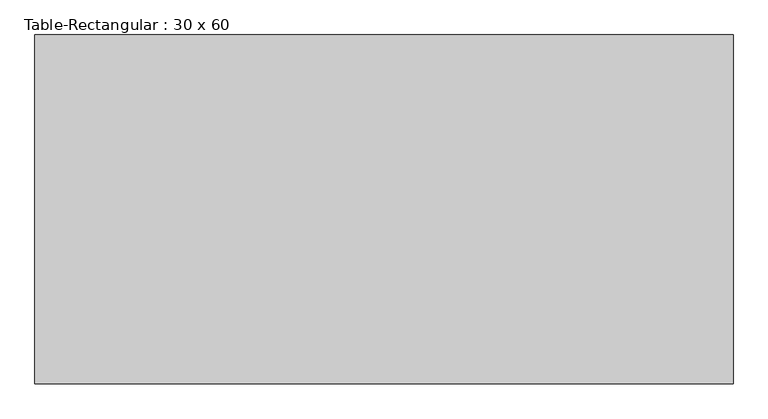
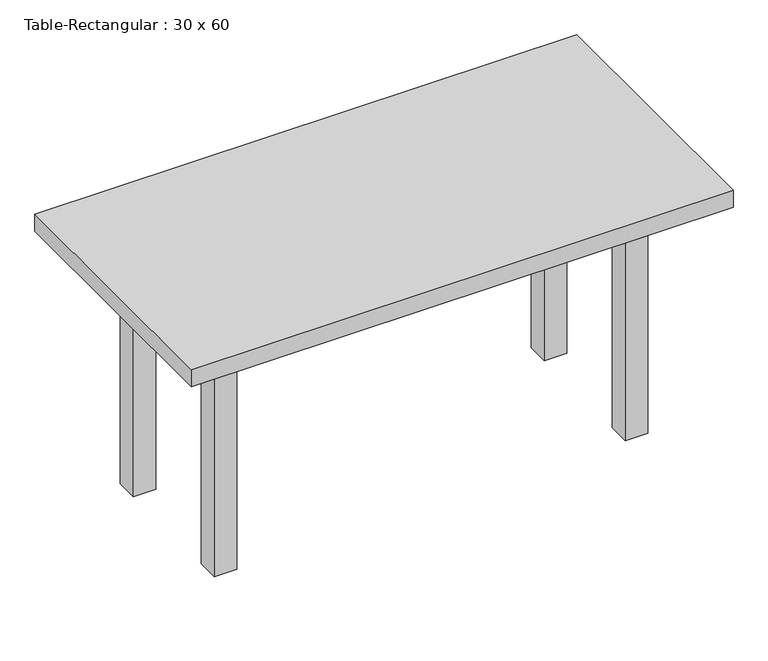
"""IFC4 building model written with IfcOpenShell, lengths in millimetres: furniture geometry, Table-Rectangular : 30 x 60."""

from ifc_helpers import new_model, si_unit, frame, origin, origin_with_axes, place, context, project, spatial, polyline, outline, extrude, source, transform, mapped, element, save


def table_rectangular_30_x_60_d900495b(model_context):
    return source(origin(), model_context, "Body", "SweptSolid", [
        extrude(outline(polyline([(546.1, 190.5), (546.1, 165.1), (-546.1, 165.1), (-546.1, 190.5), (546.1, 190.5)])), frame((0.0, 0.0, 609.6), z_axis=(0.0, 0.0, 1.0), x_axis=(1.0, 0.0, 0.0)), (0.0, 0.0, 1.0), 101.6),
        extrude(outline(polyline([(546.1, -190.5), (-546.1, -190.5), (-546.1, -165.1), (546.1, -165.1), (546.1, -190.5)])), frame((0.0, 0.0, 609.6), z_axis=(0.0, 0.0, 1.0), x_axis=(1.0, 0.0, 0.0)), (0.0, 0.0, 1.0), 101.6),
        extrude(outline(polyline([(-558.8, -165.1), (-584.2, -165.1), (-584.2, 165.1), (-558.8, 165.1), (-558.8, -165.1)])), frame((0.0, 0.0, 609.6), z_axis=(0.0, 0.0, 1.0), x_axis=(1.0, 0.0, 0.0)), (0.0, 0.0, 1.0), 101.6),
        extrude(outline(polyline([(558.8, -165.1), (558.8, 165.1), (584.2, 165.1), (584.2, -165.1), (558.8, -165.1)])), frame((0.0, 0.0, 609.6), z_axis=(0.0, 0.0, 1.0), x_axis=(1.0, 0.0, 0.0)), (0.0, 0.0, 1.0), 101.6),
        extrude(outline(polyline([(762.0, 381.0), (762.0, -381.0), (-762.0, -381.0), (-762.0, 381.0), (762.0, 381.0)])), frame((0.0, 0.0, 711.2), z_axis=(0.0, 0.0, 1.0), x_axis=(1.0, 0.0, 0.0)), (0.0, 0.0, 1.0), 50.8),
        extrude(outline(polyline([(-546.1, 228.6), (-546.1, 165.1), (-609.6, 165.1), (-609.6, 228.6), (-546.1, 228.6)])), origin_with_axes(), (0.0, 0.0, 1.0), 711.2),
        extrude(outline(polyline([(546.1, 228.6), (609.6, 228.6), (609.6, 165.1), (546.1, 165.1), (546.1, 228.6)])), origin_with_axes(), (0.0, 0.0, 1.0), 711.2),
        extrude(outline(polyline([(-546.1, -228.6), (-609.6, -228.6), (-609.6, -165.1), (-546.1, -165.1), (-546.1, -228.6)])), origin_with_axes(), (0.0, 0.0, 1.0), 711.2),
        extrude(outline(polyline([(546.1, -228.6), (546.1, -165.1), (609.6, -165.1), (609.6, -228.6), (546.1, -228.6)])), origin_with_axes(), (0.0, 0.0, 1.0), 711.2),
    ])


if __name__ == "__main__":
    model = new_model("IFC4")
    model_context = context("Model", 3, world=origin())
    ifc_project = project(units=[si_unit("LENGTHUNIT", "METRE", prefix="MILLI")], contexts=[model_context])
    site = spatial("IfcSite", under=ifc_project)
    building = spatial("IfcBuilding", under=site)
    placement = place(None, origin())
    table_rectangular_30_x_60_shape = table_rectangular_30_x_60_d900495b(model_context)
    element("IfcFurniture", 1, ObjectType="Table-Rectangular : 30 x 60", at=placement, inside=building, context=model_context, shape_type="MappedRepresentation", body=[
        mapped(table_rectangular_30_x_60_shape, transform((0.0, 0.0, 0.0), x_axis=(1.0, 0.0, 0.0), y_axis=(0.0, 1.0, 0.0), z_axis=(0.0, 0.0, 1.0))),
    ])
    save(model, "model.ifc")

# Revit data of these elements
# Type "Table-Rectangular : 30 x 60"
#   Assembly Code = "E2020200"
#   Height = 2' - 6"
#   Length = 5' - 0"
#   Width = 2' - 6"
#   Base Material = Wood - Birch
#   Top Material = Wood - Birch
#   Default Elevation = 0
# Element 1 (IfcFurniture, "Table-Rectangular : 30 x 60")
#   Materials on its faces: "Wood - Birch"
# Materials
#   "Wood - Birch": class "Unassigned", colour RGB 224 178 126, transparency 0
